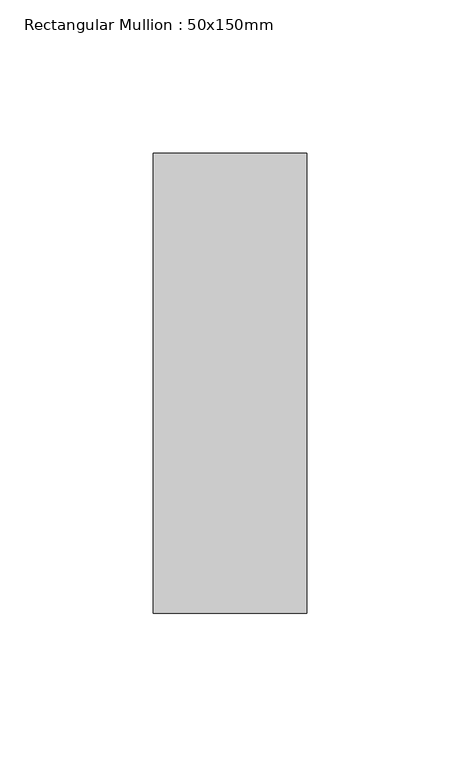
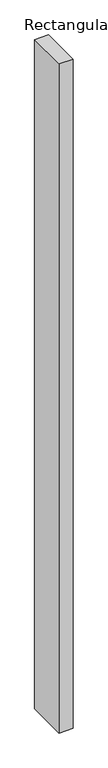
"""IFC4 building model written with IfcOpenShell, lengths in millimetres: member geometry, Rectangular Mullion : 50x150mm."""

import ifcopenshell
import ifcopenshell.guid

model = None  # the IFC model being written
_history = None  # IfcOwnerHistory: only IFC2X3 demands one
_inside = {}  # id of a spatial element -> (the spatial element, [elements in it])
_under = {}  # id of a project, library or spatial element -> (it, [spatial elements below it])
_declared = {}  # id of a project -> (the project, [libraries it declares])
_typed = {}  # id of a type object -> (the type object, [elements of that type])
_made_of = {}  # id of a material, layer set ... -> (it, [elements and type objects made of it])


def new_model(schema):
    """Start an empty IFC model of exactly this schema.

    Asked for "IFC4X3", IfcOpenShell would pick the latest addendum, in which some entities
    have other attributes; the version numbers below select the first issue.
    IFC2X3 requires an IfcOwnerHistory on every rooted entity: one is made here for all.
    """
    global model, _history
    if schema == "IFC4X3":
        model = ifcopenshell.file(schema_version=(4, 3, 0, 0))
    else:
        model = ifcopenshell.file(schema=schema)
    _inside.clear()
    _under.clear()
    _declared.clear()
    _typed.clear()
    _made_of.clear()
    _history = None
    if model.schema == "IFC2X3":
        org = make("IfcOrganization", Name="unknown")
        user = make(
            "IfcPersonAndOrganization",
            ThePerson=make("IfcPerson", FamilyName="unknown"),
            TheOrganization=org,
        )
        app = make(
            "IfcApplication",
            ApplicationDeveloper=org,
            Version="unknown",
            ApplicationFullName="unknown",
            ApplicationIdentifier="unknown",
        )
        _history = make(
            "IfcOwnerHistory",
            OwningUser=user,
            OwningApplication=app,
            ChangeAction="ADDED",
            CreationDate=0,
        )
    return model


def make(cls, **values):
    """One entity of the class cls with the attributes given. An attribute that is None is left unset."""
    return model.create_entity(
        cls, **{name: value for name, value in values.items() if value is not None}
    )


def rooted(cls, **values):
    """An entity with a GlobalId (a new one), such as an element, a storey or a relation."""
    return make(cls, GlobalId=ifcopenshell.guid.new(), OwnerHistory=_history, **values)


def si_unit(unit_type, name, prefix=None):
    """IfcSIUnit, for example si_unit("LENGTHUNIT", "METRE", prefix="MILLI")."""
    return make("IfcSIUnit", UnitType=unit_type, Prefix=prefix, Name=name)


def assignment(units):
    """IfcUnitAssignment: the units of a project."""
    return None if units is None else make("IfcUnitAssignment", Units=units)


def point(xyz):
    """IfcCartesianPoint."""
    return None if xyz is None else make("IfcCartesianPoint", Coordinates=xyz)


def direction(xyz):
    """IfcDirection."""
    return None if xyz is None else make("IfcDirection", DirectionRatios=xyz)


def frame(location, z_axis=None, x_axis=None):
    """IfcAxis2Placement3D, a coordinate frame: its origin and axes. An axis left out is left unset."""
    return make(
        "IfcAxis2Placement3D",
        Location=point(location),
        Axis=direction(z_axis),
        RefDirection=direction(x_axis),
    )


def origin():
    """The frame at (0, 0, 0) with its axes left unset."""
    return frame((0.0, 0.0, 0.0))


def place(relative_to, where):
    """IfcLocalPlacement: puts the frame where relative to a parent placement (None: the world)."""
    return make(
        "IfcLocalPlacement", PlacementRelTo=relative_to, RelativePlacement=where
    )


def context(
    kind, dimensions, precision=None, world=None, true_north=None, identifier=None
):
    """IfcGeometricRepresentationContext, for example the 3D "Model" context."""
    return make(
        "IfcGeometricRepresentationContext",
        ContextIdentifier=identifier,
        ContextType=kind,
        CoordinateSpaceDimension=dimensions,
        Precision=precision,
        WorldCoordinateSystem=world,
        TrueNorth=true_north,
    )


def project(units=None, contexts=None):
    """IfcProject with its units and contexts."""
    return rooted(
        "IfcProject",
        Name="project",
        RepresentationContexts=contexts,
        UnitsInContext=assignment(units),
    )


def spatial(cls, under=None, at=None, **own):
    """A site, building, storey or space (cls), placed at a placement, below another one or the project."""
    s = rooted(cls, ObjectPlacement=at, **own)
    if under is not None:
        _under.setdefault(under.id(), (under, []))[1].append(s)
    return s


def polyline(points):
    """IfcPolyline through the points."""
    return make("IfcPolyline", Points=[point(p) for p in points])


def outline(outer, holes=None, kind="AREA"):
    """IfcArbitraryClosedProfileDef: a profile drawn as a closed curve; with holes, ...WithVoids."""
    if holes is None:
        return make("IfcArbitraryClosedProfileDef", ProfileType=kind, OuterCurve=outer)
    return make(
        "IfcArbitraryProfileDefWithVoids",
        ProfileType=kind,
        OuterCurve=outer,
        InnerCurves=holes,
    )


def extrude(swept, where, along, depth):
    """IfcExtrudedAreaSolid: the profile swept, set in the frame where, extruded along a direction by depth."""
    return make(
        "IfcExtrudedAreaSolid",
        SweptArea=swept,
        Position=where,
        ExtrudedDirection=direction(along),
        Depth=depth,
    )


def shape(context_of_items, identifier, shape_type, items):
    """IfcShapeRepresentation: the items that make up one representation, for example the "Body"."""
    return make(
        "IfcShapeRepresentation",
        ContextOfItems=context_of_items,
        RepresentationIdentifier=identifier,
        RepresentationType=shape_type,
        Items=items,
    )


def source(mapping_origin, context_of_items, identifier, shape_type, items):
    """IfcRepresentationMap: a shape defined once, which mapped items show again and again."""
    return make(
        "IfcRepresentationMap",
        MappingOrigin=mapping_origin,
        MappedRepresentation=shape(context_of_items, identifier, shape_type, items),
    )


def transform(
    local_origin,
    x_axis=None,
    y_axis=None,
    z_axis=None,
    scale=None,
    scale2=None,
    scale3=None,
    uniform=True,
):
    """IfcCartesianTransformationOperator3D, or its non-uniform kind. x_axis, y_axis, z_axis: its Axis1, 2, 3."""
    if uniform:
        return make(
            "IfcCartesianTransformationOperator3D",
            Axis1=direction(x_axis),
            Axis2=direction(y_axis),
            LocalOrigin=point(local_origin),
            Scale=scale,
            Axis3=direction(z_axis),
        )
    return make(
        "IfcCartesianTransformationOperator3DnonUniform",
        Axis1=direction(x_axis),
        Axis2=direction(y_axis),
        LocalOrigin=point(local_origin),
        Scale=scale,
        Axis3=direction(z_axis),
        Scale2=scale2,
        Scale3=scale3,
    )


def mapped(mapping_source, mapping_target):
    """IfcMappedItem: shows the shape of a source again, moved by a transform."""
    return make(
        "IfcMappedItem", MappingSource=mapping_source, MappingTarget=mapping_target
    )


def made_of(thing, what):
    """Note that an element or type object is made of a material, layer set ...; save() writes the relation."""
    if what is not None:
        _made_of.setdefault(what.id(), (what, []))[1].append(thing)
    return thing


def element(
    cls,
    number,
    at=None,
    inside=None,
    cuts=None,
    type_object=None,
    material=None,
    context=None,
    identifier="Body",
    shape_type=None,
    held_by="IfcProductDefinitionShape",
    body=None,
    shapes=None,
    **own,
):
    """One element of the class cls, such as IfcWall. Its Tag is "e" and its number.

    at: its placement. inside: the storey or other place that contains it. cuts: it is an
    opening in that element (IfcRelVoidsElement). A single representation is given by context,
    identifier, shape_type and body (its items); several are given by shapes. held_by: the class
    of the entity that holds the representations. save() writes the other relations.
    """
    e = rooted(cls, Tag="e%d" % number, ObjectPlacement=at, **own)
    if body is not None:
        shapes = [shape(context, identifier, shape_type, body)]
    if shapes is not None:
        e.Representation = make(held_by, Representations=shapes)
    if inside is not None:
        _inside.setdefault(inside.id(), (inside, []))[1].append(e)
    if cuts is not None:
        rooted(
            "IfcRelVoidsElement", RelatingBuildingElement=cuts, RelatedOpeningElement=e
        )
    if type_object is not None:
        _typed.setdefault(type_object.id(), (type_object, []))[1].append(e)
    return made_of(e, material)


def aggregate(whole, parts):
    """IfcRelAggregates: a whole, such as a stair, and the parts it consists of."""
    return rooted("IfcRelAggregates", RelatingObject=whole, RelatedObjects=parts)


def save(model, path):
    """Write the relations noted so far, then the file.

    IfcRelAggregates (storeys below a building ...), IfcRelContainedInSpatialStructure (elements
    in a storey), IfcRelDefinesByType, IfcRelAssociatesMaterial and IfcRelDeclares: one each for
    every whole, place, type object, material and project.
    """
    for whole, parts in _under.values():
        aggregate(whole, parts)
    for where, things in _inside.values():
        rooted(
            "IfcRelContainedInSpatialStructure",
            RelatedElements=things,
            RelatingStructure=where,
        )
    for kind, things in _typed.values():
        rooted("IfcRelDefinesByType", RelatedObjects=things, RelatingType=kind)
    for what, things in _made_of.values():
        rooted("IfcRelAssociatesMaterial", RelatedObjects=things, RelatingMaterial=what)
    for by, libraries in _declared.values():
        rooted("IfcRelDeclares", RelatingContext=by, RelatedDefinitions=libraries)
    model.write(path)


def rectangular_mullion_50x150mm_5d7d41ff(model_context):
    return source(origin(), model_context, "Body", "SweptSolid", [
        extrude(outline(polyline([(25.0, 75.0), (25.0, -75.0), (-25.0, -75.0), (-25.0, 75.0), (25.0, 75.0)])), frame((0.0, 0.0, -2522.0381538), z_axis=(0.0, 0.0, 1.0), x_axis=(1.0, 0.0, 0.0)), (0.0, 0.0, 1.0), 2522.0381538),
    ])


if __name__ == "__main__":
    model = new_model("IFC4")
    model_context = context("Model", 3, world=origin())
    ifc_project = project(units=[si_unit("LENGTHUNIT", "METRE", prefix="MILLI")], contexts=[model_context])
    site = spatial("IfcSite", under=ifc_project)
    building = spatial("IfcBuilding", under=site)
    placement = place(None, origin())
    rectangular_mullion_50x150mm_shape = rectangular_mullion_50x150mm_5d7d41ff(model_context)
    element("IfcMember", 1, ObjectType="Rectangular Mullion : 50x150mm", at=placement, inside=building, context=model_context, shape_type="MappedRepresentation", body=[
        mapped(rectangular_mullion_50x150mm_shape, transform((0.0, 0.0, 0.0), x_axis=(1.0, 0.0, 0.0), y_axis=(0.0, 1.0, 0.0), z_axis=(0.0, 0.0, 1.0))),
    ])
    save(model, "model.ifc")

# Revit data of these elements
# Type "Rectangular Mullion : 50x150mm"
#   Keynote = "H11"
#   built-in parameter 1007304 = 0.492126 (stored number, unit not read)
#   built-in parameter 1007301 = 0.082021 (stored number, unit not read)
#   built-in parameter 1007300 = 0.082021 (stored number, unit not read)
# Element 1 (IfcMember, "Rectangular Mullion : 50x150mm")
#   Materials on its faces: "Aluminium"
# Materials
#   "Aluminium": class "Metal", colour RGB 247 247 247, transparency 0, Description = "Aluminium 6061", Cost = 0
